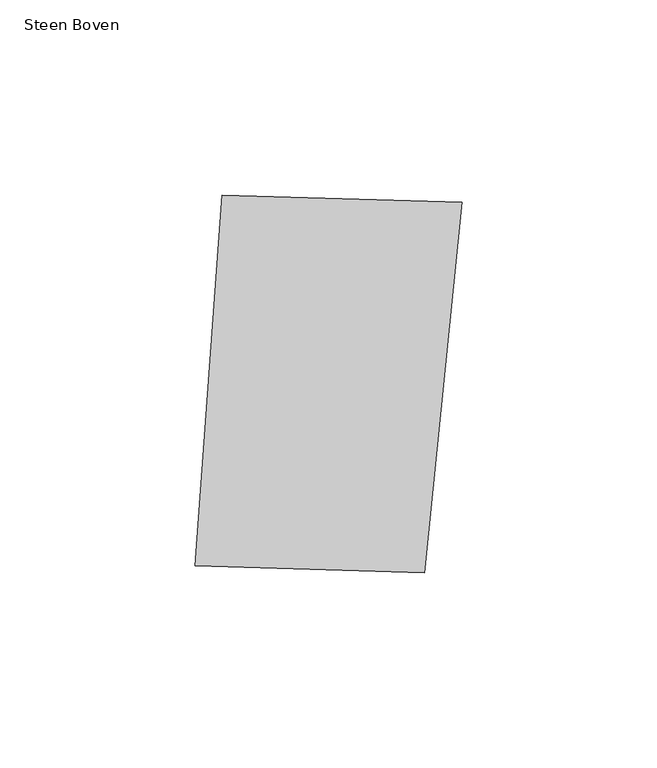
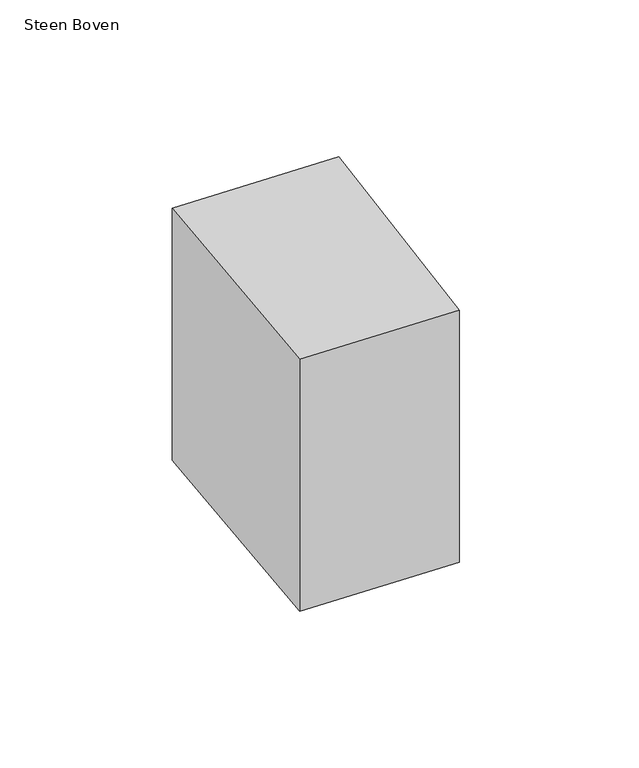
"""IFC4 building model written with IfcOpenShell, lengths in millimetres: proxy geometry, 00_GMA_steen_versie_4 : Steen Boven."""

from ifc_helpers import new_model, si_unit, origin, origin_with_axes, place, context, project, spatial, polyline, outline, extrude, source, transform, mapped, element, save


def steen_boven_c53dbaa5(model_context):
    return source(origin(), model_context, "Body", "SweptSolid", [
        extrude(outline(polyline([(105.6135856, 118.6166658), (96.0016628, 23.8486793), (37.3143143, 25.6033935), (44.212237, 120.4452637), (105.6135856, 118.6166658)])), origin_with_axes(), (0.0, 0.0, 1.0), 100.0),
    ])


if __name__ == "__main__":
    model = new_model("IFC4")
    model_context = context("Model", 3, world=origin())
    ifc_project = project(units=[si_unit("LENGTHUNIT", "METRE", prefix="MILLI")], contexts=[model_context])
    site = spatial("IfcSite", under=ifc_project)
    building = spatial("IfcBuilding", under=site)
    placement = place(None, origin())
    steen_boven_shape = steen_boven_c53dbaa5(model_context)
    element("IfcBuildingElementProxy", 1, Name="00_GMA_steen_versie_4 : Steen Boven", ObjectType="00_GMA_steen_versie_4 : Steen Boven", at=placement, inside=building, context=model_context, shape_type="MappedRepresentation", body=[
        mapped(steen_boven_shape, transform((0.0, 0.0, 0.0), x_axis=(1.0, 0.0, 0.0), y_axis=(0.0, 1.0, 0.0), z_axis=(0.0, 0.0, 1.0))),
    ])
    save(model, "model.ifc")

# Revit data of these elements
# Type "00_GMA_steen_versie_4 : Steen Boven"
#   StootVoegHalfBoven [instance default] = 5 mm
#   StootVoegHalf [instance default] = 5 mm
#   StootVoegBreedteOnder = 10 mm
#   StootVoegBreedteBoven = 10 mm
#   Steendikte = 100 mm
#   LintVoegOnderHalf = 5 mm
#   LintVoegOnder = 10 mm
#   LintVoegBovenHalf = 0 mm
#   LintVoegBoven = 0 mm
#   materiaal = none
#   MateriaalVoeg = none
#   Default Elevation = 0
